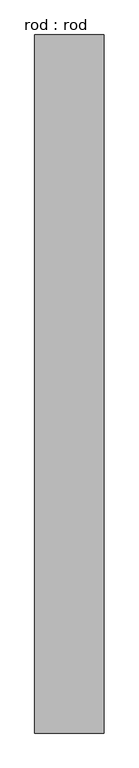
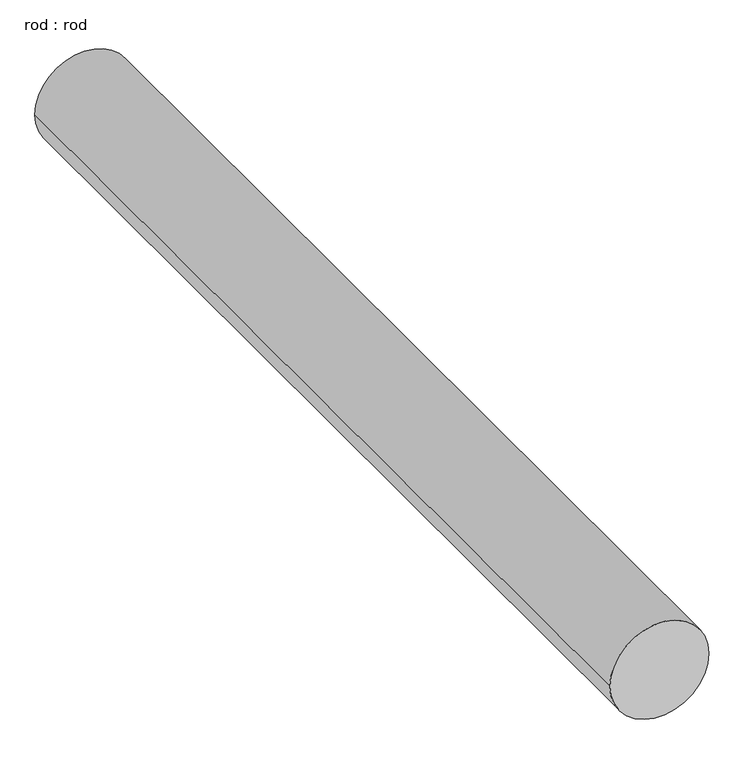
"""IFC4 building model written with IfcOpenShell, lengths in millimetres: proxy geometry, rod : rod."""

from ifc_helpers import new_model, si_unit, point, frame, frame_2d, origin, place, context, project, spatial, circle_curve, trimmed, segment, composite_curve, outline, extrude, source, transform, mapped, element, save


def rod_rod_0db02414(model_context):
    return source(origin(), model_context, "Body", "SweptSolid", [
        extrude(outline(composite_curve([segment(trimmed(circle_curve(frame_2d((0.0108462, 0.0)), 200.0), [point((0.0108462, 200.0))], [point((0.0108462, -200.0))], False, "CARTESIAN"), True, "CONTINUOUS"), segment(trimmed(circle_curve(frame_2d((0.0108462, 0.0)), 200.0), [point((0.0108462, -200.0))], [point((0.0108462, 200.0))], False, "CARTESIAN"), True, "CONTINUOUS")], self_intersect=False)), frame((0.0, 2081.3220801, 0.0), z_axis=(0.0, 1.0, 0.0), x_axis=(0.0, 0.0, 1.0)), (0.0, 0.0, 1.0), 4022.8130705),
    ])


if __name__ == "__main__":
    model = new_model("IFC4")
    model_context = context("Model", 3, world=origin())
    ifc_project = project(units=[si_unit("LENGTHUNIT", "METRE", prefix="MILLI")], contexts=[model_context])
    site = spatial("IfcSite", under=ifc_project)
    building = spatial("IfcBuilding", under=site)
    placement = place(None, origin())
    rod_rod_shape = rod_rod_0db02414(model_context)
    element("IfcBuildingElementProxy", 1, Name="rod : rod", ObjectType="rod : rod", at=placement, inside=building, context=model_context, shape_type="MappedRepresentation", body=[
        mapped(rod_rod_shape, transform((0.0, 0.0, 0.0), x_axis=(1.0, 0.0, 0.0), y_axis=(0.0, 1.0, 0.0), z_axis=(0.0, 0.0, 1.0))),
    ])
    save(model, "model.ifc")

# Revit data of these elements
# Type "rod : rod"
#   Default Elevation = 0
